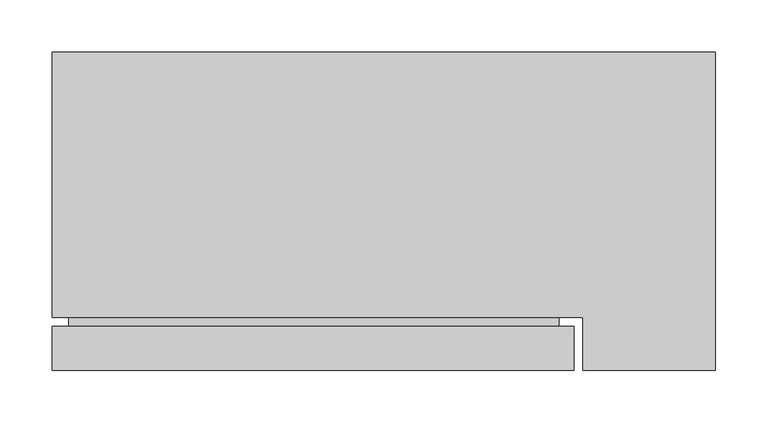
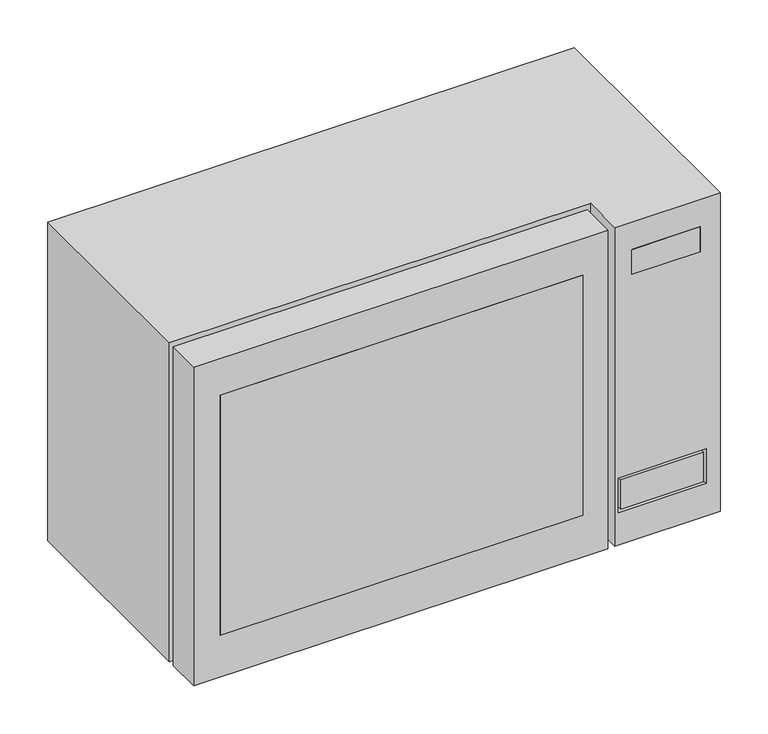
"""IFC4 building model written with IfcOpenShell, lengths in millimetres: proxy geometry, Microwave, Under Cabinet - NON-COLLECTUS : -."""

from ifc_helpers import new_model, si_unit, frame, origin, place, context, project, spatial, polyline, outline, extrude, faceted_brep, source, transform, mapped, element, save


def specialty_equipment_66306a0b(model_context):
    return source(origin(), model_context, "Body", "SolidModel", [
        extrude(outline(polyline([(293.2332881, -152.4), (210.6832881, -152.4), (210.6832881, -146.05), (293.2332881, -146.05), (293.2332881, -152.4)])), frame((0.0, 0.0, 339.67213), z_axis=(0.0, 0.0, 1.0), x_axis=(1.0, 0.0, 0.0)), (0.0, 0.0, 1.0), 31.75),
        extrude(outline(polyline([(151.7767768, -152.4), (-285.75, -152.4), (-285.75, -146.05), (151.7767768, -146.05), (151.7767768, -152.4)])), frame((0.0, 0.0, 53.1848179), z_axis=(0.0, 0.0, 1.0), x_axis=(1.0, 0.0, 0.0)), (0.0, 0.0, 1.0), 306.0096891),
        faceted_brep([(-317.5, -110.0756803, 406.4), (-317.5, -152.4, 406.4), (181.8942849, -152.4, 406.4), (181.8942849, -110.0756803, 406.4), (-317.5, -110.0756803, 0.0), (181.8942849, -110.0756803, 0.0), (181.8942849, -152.4, 0.0), (-317.5, -152.4, 0.0), (-285.75, -152.4, 359.194507), (151.7767768, -152.4, 359.194507), (151.7767768, -152.4, 53.1848179), (-285.75, -152.4, 53.1848179), (151.7767768, -146.05, 359.194507), (-285.75, -146.05, 359.194507), (-285.75, -146.05, 53.1848179), (151.7767768, -146.05, 53.1848179)], [[[0, 1, 2, 3]], [[4, 5, 6, 7]], [[1, 0, 4, 7]], [[2, 1, 7, 6], [8, 9, 10, 11]], [[3, 2, 6, 5]], [[0, 3, 5, 4]], [[12, 13, 14, 15]], [[13, 12, 9, 8]], [[14, 13, 8, 11]], [[15, 14, 11, 10]], [[12, 15, 10, 9]]]),
        extrude(outline(polyline([(-301.7486762, -101.6), (167.8090947, -101.6), (167.8090947, -110.0756803), (-301.7486762, -110.0756803), (-301.7486762, -101.6)])), frame((0.0, 0.0, 38.5670061), z_axis=(0.0, 0.0, 1.0), x_axis=(1.0, 0.0, 0.0)), (0.0, 0.0, 1.0), 339.6775009),
        faceted_brep([(317.5, 152.4, 406.4), (-317.5, 152.4, 406.4), (-317.5, -101.6, 406.4), (190.5, -101.6, 406.4), (190.5, -152.4, 406.4), (317.5, -152.4, 406.4), (317.5, 152.4, 0.0), (317.5, -152.4, 0.0), (190.5, -152.4, 0.0), (190.5, -101.6, 0.0), (-317.5, -101.6, 0.0), (-317.5, 152.4, 0.0), (210.6832881, -152.4, 371.42213), (293.2332881, -152.4, 371.42213), (293.2332881, -152.4, 339.67213), (210.6832881, -152.4, 339.67213), (300.6704981, -152.4, 41.6136485), (194.5902288, -152.4, 41.6136485), (194.5902288, -152.4, 85.6060767), (300.6704981, -152.4, 85.6060767), (297.3748845, -152.4, 82.3104632), (197.8858423, -152.4, 82.3104632), (197.8858423, -152.4, 44.909262), (297.3748845, -152.4, 44.909262), (293.2332881, -146.05, 371.42213), (210.6832881, -146.05, 371.42213), (210.6832881, -146.05, 339.67213), (293.2332881, -146.05, 339.67213), (297.3748845, -146.05, 85.6060767), (197.8858423, -146.05, 85.6060767), (197.8858423, -146.05, 82.3104632), (297.3748845, -146.05, 82.3104632), (297.3748845, -133.4626171, 85.6060767), (300.6704981, -133.4626171, 85.6060767), (194.5902288, -133.4626171, 85.6060767), (197.8858423, -133.4626171, 85.6060767), (297.3748845, -133.4626171, 44.909262), (197.8858423, -133.4626171, 44.909262), (194.5902288, -133.4626171, 41.6136485), (300.6704981, -133.4626171, 41.6136485)], [[[0, 1, 2, 3, 4, 5]], [[6, 7, 8, 9, 10, 11]], [[1, 0, 6, 11]], [[2, 1, 11, 10]], [[3, 2, 10, 9]], [[4, 3, 9, 8]], [[5, 4, 8, 7], [12, 13, 14, 15], [16, 17, 18, 19]], [[20, 21, 22, 23]], [[0, 5, 7, 6]], [[24, 25, 26, 27]], [[25, 24, 13, 12]], [[26, 25, 12, 15]], [[27, 26, 15, 14]], [[24, 27, 14, 13]], [[28, 29, 30, 31]], [[29, 28, 32, 33, 19, 18, 34, 35]], [[31, 30, 21, 20]], [[36, 37, 35, 34, 38, 39, 33, 32]], [[37, 36, 23, 22]], [[39, 38, 17, 16]], [[38, 34, 18, 17]], [[29, 35, 37, 22, 21, 30]], [[32, 28, 31, 20, 23, 36]], [[33, 39, 16, 19]]]),
    ])


if __name__ == "__main__":
    model = new_model("IFC4")
    model_context = context("Model", 3, world=origin())
    ifc_project = project(units=[si_unit("LENGTHUNIT", "METRE", prefix="MILLI")], contexts=[model_context])
    site = spatial("IfcSite", under=ifc_project)
    building = spatial("IfcBuilding", under=site)
    placement = place(None, origin())
    specialty_equipment_shape = specialty_equipment_66306a0b(model_context)
    element("IfcBuildingElementProxy", 1, Name="Microwave, Under Cabinet - NON-COLLECTUS : -", ObjectType="Microwave, Under Cabinet - NON-COLLECTUS : -", at=placement, inside=building, context=model_context, shape_type="MappedRepresentation", body=[
        mapped(specialty_equipment_shape, transform((0.0, 0.0, 0.0), x_axis=(1.0, 0.0, 0.0), y_axis=(0.0, 1.0, 0.0), z_axis=(0.0, 0.0, 1.0))),
    ])
    save(model, "model.ifc")

# Revit data of these elements
# Type "Microwave, Under Cabinet - NON-COLLECTUS : -"
#   External ID [instance default] = ""
#   Width = 635 mm
#   Height = 406.4 mm
#   Depth = 304.8 mm
#   Material = Light Grey
#   Default Elevation = 0
# Element 1 (IfcBuildingElementProxy, "Microwave, Under Cabinet - NON-COLLECTUS : -")
#   Materials on its faces: "Light Grey"
# Materials
#   "Light Grey": class "Generic", colour RGB 215 215 215, transparency 0, Cost = 0
